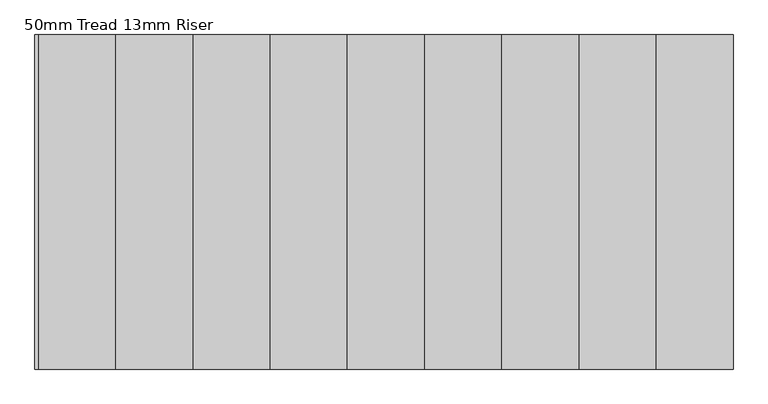
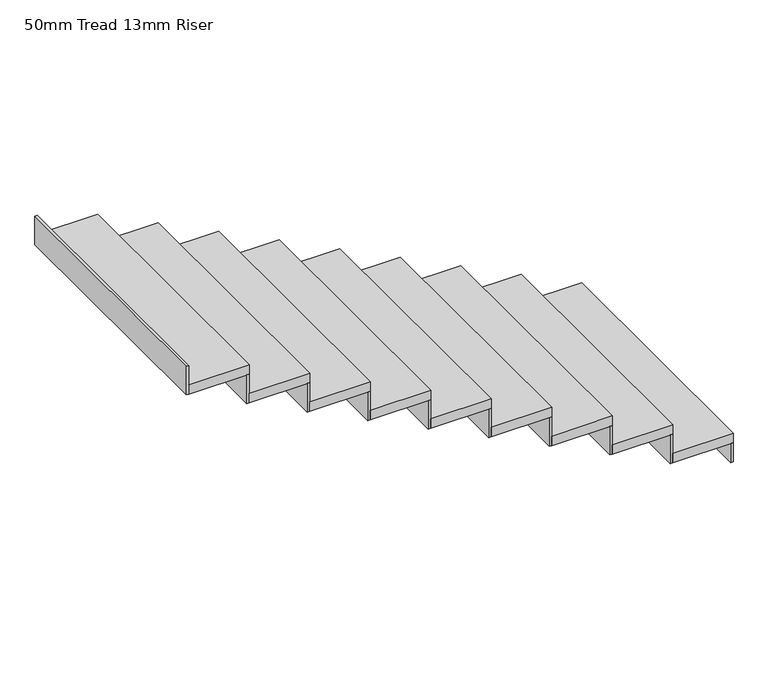
"""IFC4 building model written with IfcOpenShell, lengths in millimetres: stair flight geometry, 50mm Tread 13mm Riser."""

from ifc_helpers import new_model, si_unit, frame, origin, origin_with_axes, place, context, project, spatial, polyline, outline, extrude, source, transform, mapped, element, save


def stair_flight_50mm_tread_13mm_riser_07300590(model_context):
    return source(origin(), model_context, "Body", "SweptSolid", [
        extrude(outline(polyline([(-10508.0859635, -1821.1593564), (-10495.5859635, -1821.1593564), (-10495.5859635, -3121.1593564), (-10508.0859635, -3121.1593564), (-10508.0859635, -1821.1593564)])), origin_with_axes(), (0.0, 0.0, 1.0), 100.0),
        extrude(outline(polyline([(-10795.5859635, -3121.1593564), (-10795.5859635, -1821.1593564), (-10495.5859635, -1821.1593564), (-10495.5859635, -3121.1593564), (-10795.5859635, -3121.1593564)])), frame((0.0, 0.0, 100.0), z_axis=(0.0, 0.0, 1.0), x_axis=(1.0, 0.0, 0.0)), (0.0, 0.0, 1.0), 50.0),
        extrude(outline(polyline([(-10808.0859635, -1821.1593564), (-10795.5859635, -1821.1593564), (-10795.5859635, -3121.1593564), (-10808.0859635, -3121.1593564), (-10808.0859635, -1821.1593564)])), frame((0.0, 0.0, 100.0), z_axis=(0.0, 0.0, 1.0), x_axis=(1.0, 0.0, 0.0)), (0.0, 0.0, 1.0), 150.0),
        extrude(outline(polyline([(-11095.5859635, -3121.1593564), (-11095.5859635, -1821.1593564), (-10795.5859635, -1821.1593564), (-10795.5859635, -3121.1593564), (-11095.5859635, -3121.1593564)])), frame((0.0, 0.0, 250.0), z_axis=(0.0, 0.0, 1.0), x_axis=(1.0, 0.0, 0.0)), (0.0, 0.0, 1.0), 50.0),
        extrude(outline(polyline([(-11108.0859635, -1821.1593564), (-11095.5859635, -1821.1593564), (-11095.5859635, -3121.1593564), (-11108.0859635, -3121.1593564), (-11108.0859635, -1821.1593564)])), frame((0.0, 0.0, 250.0), z_axis=(0.0, 0.0, 1.0), x_axis=(1.0, 0.0, 0.0)), (0.0, 0.0, 1.0), 150.0),
        extrude(outline(polyline([(-11395.5859635, -3121.1593564), (-11395.5859635, -1821.1593564), (-11095.5859635, -1821.1593564), (-11095.5859635, -3121.1593564), (-11395.5859635, -3121.1593564)])), frame((0.0, 0.0, 400.0), z_axis=(0.0, 0.0, 1.0), x_axis=(1.0, 0.0, 0.0)), (0.0, 0.0, 1.0), 50.0),
        extrude(outline(polyline([(-11408.0859635, -1821.1593564), (-11395.5859635, -1821.1593564), (-11395.5859635, -3121.1593564), (-11408.0859635, -3121.1593564), (-11408.0859635, -1821.1593564)])), frame((0.0, 0.0, 400.0), z_axis=(0.0, 0.0, 1.0), x_axis=(1.0, 0.0, 0.0)), (0.0, 0.0, 1.0), 150.0),
        extrude(outline(polyline([(-11695.5859635, -3121.1593564), (-11695.5859635, -1821.1593564), (-11395.5859635, -1821.1593564), (-11395.5859635, -3121.1593564), (-11695.5859635, -3121.1593564)])), frame((0.0, 0.0, 550.0), z_axis=(0.0, 0.0, 1.0), x_axis=(1.0, 0.0, 0.0)), (0.0, 0.0, 1.0), 50.0),
        extrude(outline(polyline([(-11708.0859635, -1821.1593564), (-11695.5859635, -1821.1593564), (-11695.5859635, -3121.1593564), (-11708.0859635, -3121.1593564), (-11708.0859635, -1821.1593564)])), frame((0.0, 0.0, 550.0), z_axis=(0.0, 0.0, 1.0), x_axis=(1.0, 0.0, 0.0)), (0.0, 0.0, 1.0), 150.0),
        extrude(outline(polyline([(-11995.5859635, -3121.1593564), (-11995.5859635, -1821.1593564), (-11695.5859635, -1821.1593564), (-11695.5859635, -3121.1593564), (-11995.5859635, -3121.1593564)])), frame((0.0, 0.0, 700.0), z_axis=(0.0, 0.0, 1.0), x_axis=(1.0, 0.0, 0.0)), (0.0, 0.0, 1.0), 50.0),
        extrude(outline(polyline([(-12008.0859635, -1821.1593564), (-11995.5859635, -1821.1593564), (-11995.5859635, -3121.1593564), (-12008.0859635, -3121.1593564), (-12008.0859635, -1821.1593564)])), frame((0.0, 0.0, 700.0), z_axis=(0.0, 0.0, 1.0), x_axis=(1.0, 0.0, 0.0)), (0.0, 0.0, 1.0), 150.0),
        extrude(outline(polyline([(-12295.5859635, -3121.1593564), (-12295.5859635, -1821.1593564), (-11995.5859635, -1821.1593564), (-11995.5859635, -3121.1593564), (-12295.5859635, -3121.1593564)])), frame((0.0, 0.0, 850.0), z_axis=(0.0, 0.0, 1.0), x_axis=(1.0, 0.0, 0.0)), (0.0, 0.0, 1.0), 50.0),
        extrude(outline(polyline([(-12308.0859635, -1821.1593564), (-12295.5859635, -1821.1593564), (-12295.5859635, -3121.1593564), (-12308.0859635, -3121.1593564), (-12308.0859635, -1821.1593564)])), frame((0.0, 0.0, 850.0), z_axis=(0.0, 0.0, 1.0), x_axis=(1.0, 0.0, 0.0)), (0.0, 0.0, 1.0), 150.0),
        extrude(outline(polyline([(-12595.5859635, -3121.1593564), (-12595.5859635, -1821.1593564), (-12295.5859635, -1821.1593564), (-12295.5859635, -3121.1593564), (-12595.5859635, -3121.1593564)])), frame((0.0, 0.0, 1000.0), z_axis=(0.0, 0.0, 1.0), x_axis=(1.0, 0.0, 0.0)), (0.0, 0.0, 1.0), 50.0),
        extrude(outline(polyline([(-12608.0859635, -1821.1593564), (-12595.5859635, -1821.1593564), (-12595.5859635, -3121.1593564), (-12608.0859635, -3121.1593564), (-12608.0859635, -1821.1593564)])), frame((0.0, 0.0, 1000.0), z_axis=(0.0, 0.0, 1.0), x_axis=(1.0, 0.0, 0.0)), (0.0, 0.0, 1.0), 150.0),
        extrude(outline(polyline([(-12895.5859635, -3121.1593564), (-12895.5859635, -1821.1593564), (-12595.5859635, -1821.1593564), (-12595.5859635, -3121.1593564), (-12895.5859635, -3121.1593564)])), frame((0.0, 0.0, 1150.0), z_axis=(0.0, 0.0, 1.0), x_axis=(1.0, 0.0, 0.0)), (0.0, 0.0, 1.0), 50.0),
        extrude(outline(polyline([(-12908.0859635, -1821.1593564), (-12895.5859635, -1821.1593564), (-12895.5859635, -3121.1593564), (-12908.0859635, -3121.1593564), (-12908.0859635, -1821.1593564)])), frame((0.0, 0.0, 1150.0), z_axis=(0.0, 0.0, 1.0), x_axis=(1.0, 0.0, 0.0)), (0.0, 0.0, 1.0), 150.0),
        extrude(outline(polyline([(-13208.0859635, -1821.1593564), (-13195.5859635, -1821.1593564), (-13195.5859635, -3121.1593564), (-13208.0859635, -3121.1593564), (-13208.0859635, -1821.1593564)])), frame((0.0, 0.0, 1300.0), z_axis=(0.0, 0.0, 1.0), x_axis=(1.0, 0.0, 0.0)), (0.0, 0.0, 1.0), 150.0),
        extrude(outline(polyline([(-13195.5859635, -3121.1593564), (-13195.5859635, -1821.1593564), (-12895.5859635, -1821.1593564), (-12895.5859635, -3121.1593564), (-13195.5859635, -3121.1593564)])), frame((0.0, 0.0, 1300.0), z_axis=(0.0, 0.0, 1.0), x_axis=(1.0, 0.0, 0.0)), (0.0, 0.0, 1.0), 50.0),
    ])


if __name__ == "__main__":
    model = new_model("IFC4")
    model_context = context("Model", 3, world=origin())
    ifc_project = project(units=[si_unit("LENGTHUNIT", "METRE", prefix="MILLI")], contexts=[model_context])
    site = spatial("IfcSite", under=ifc_project)
    building = spatial("IfcBuilding", under=site)
    placement = place(None, origin())
    stair_flight_50mm_tread_13mm_riser_shape = stair_flight_50mm_tread_13mm_riser_07300590(model_context)
    element("IfcStairFlight", 1, ObjectType="50mm Tread 13mm Riser", at=placement, inside=building, context=model_context, shape_type="MappedRepresentation", body=[
        mapped(stair_flight_50mm_tread_13mm_riser_shape, transform((0.0, 0.0, 0.0), x_axis=(1.0, 0.0, 0.0), y_axis=(0.0, 1.0, 0.0), z_axis=(0.0, 0.0, 1.0))),
    ])
    save(model, "model.ifc")
